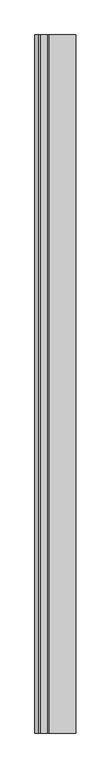
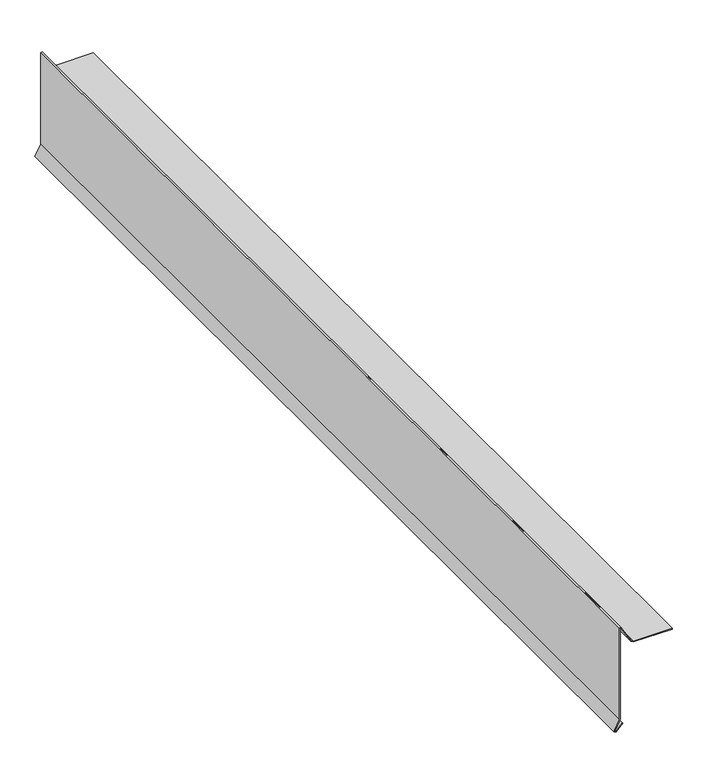
"""IFC4 building model written with IfcOpenShell, lengths in millimetres: proxy geometry, GRAVEL STOP006 14641 : GRAVEL STOP006 14641."""

from ifc_helpers import new_model, si_unit, frame, origin, place, context, project, spatial, polyline, outline, extrude, source, transform, mapped, element, save


def generic_models_072a6e35(model_context):
    return source(origin(), model_context, "Body", "SweptSolid", [
        extrude(outline(polyline([(40077.410403, -2814.9855343), (40091.8049, -2800.5910374), (40092.8027062, -2801.5888435), (40079.2807815, -2815.1107682), (40080.9054201, -2817.2404183), (40101.495749, -2805.9993985), (40293.447969, -2805.9993985), (40293.699878, -2805.0592614), (40258.5078708, -2784.7411466), (40255.9633674, -2780.3339375), (40255.9633674, -2702.4979247), (40257.3744784, -2702.4979247), (40257.3744784, -2779.9558314), (40259.5408757, -2783.7081416), (40295.3431515, -2804.3785952), (40294.5307525, -2807.4105095), (40101.8558531, -2807.4105095), (40080.5182783, -2819.0594785), (40077.410403, -2814.9855343)])), frame((0.0, 999.75, 0.0), z_axis=(0.0, 1.0, 0.0), x_axis=(0.0, 0.0, 1.0)), (0.0, 0.0, 1.0), 2000.25),
    ])


if __name__ == "__main__":
    model = new_model("IFC4")
    model_context = context("Model", 3, world=origin())
    ifc_project = project(units=[si_unit("LENGTHUNIT", "METRE", prefix="MILLI")], contexts=[model_context])
    site = spatial("IfcSite", under=ifc_project)
    building = spatial("IfcBuilding", under=site)
    placement = place(None, origin())
    generic_models_shape = generic_models_072a6e35(model_context)
    element("IfcBuildingElementProxy", 1, Name="GRAVEL STOP006 14641 : GRAVEL STOP006 14641", ObjectType="GRAVEL STOP006 14641 : GRAVEL STOP006 14641", at=placement, inside=building, context=model_context, shape_type="MappedRepresentation", body=[
        mapped(generic_models_shape, transform((0.0, 0.0, 0.0), x_axis=(1.0, 0.0, 0.0), y_axis=(0.0, 1.0, 0.0), z_axis=(0.0, 0.0, 1.0))),
    ])
    save(model, "model.ifc")

# Revit data of these elements
# Type "GRAVEL STOP006 14641 : GRAVEL STOP006 14641"
#   NameOverride = "GRAVEL STOP006"
# Element 1 (IfcBuildingElementProxy, "GRAVEL STOP006 14641 : GRAVEL STOP006 14641")
#   Materials on its faces: "GRAVEL STOP REQUIRED WITH GRAVEL SURFACE SYSTEMS"
# Materials
#   "GRAVEL STOP REQUIRED WITH GRAVEL SURFACE SYSTEMS": class "Unassigned", colour RGB 170 170 127, transparency 0
